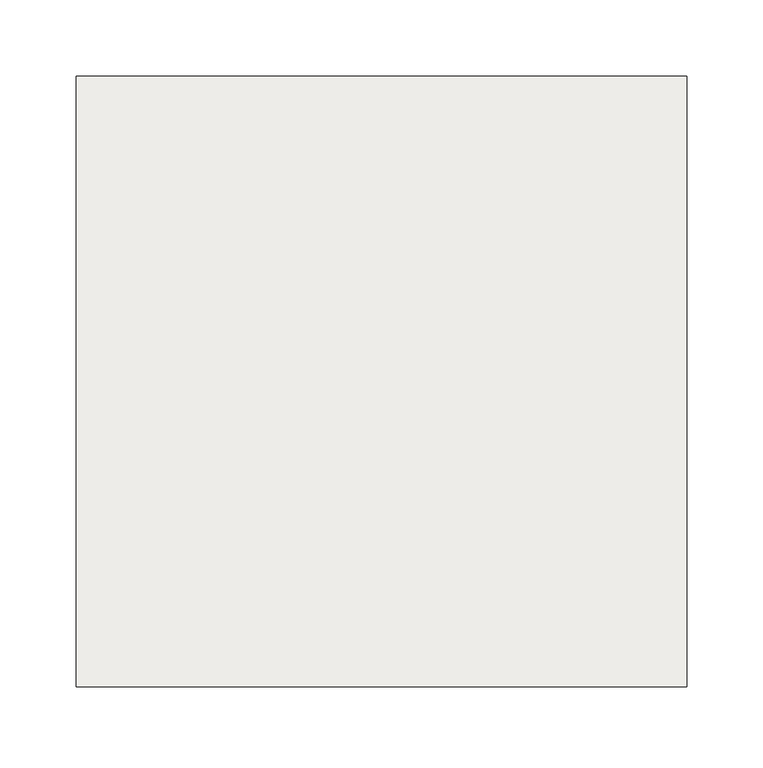
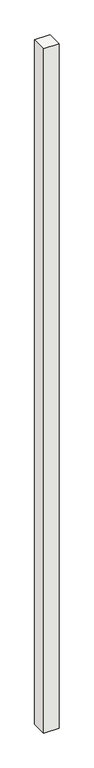
"""IFC4 building model written with IfcOpenShell, lengths in millimetres: footing geometry, NLRS_17_SFO_TLB_funderingspaal geheid beton prefab-AV-MMBPC_gen_rsf : heipaal beton prefab_gen__bxh 400x400."""

from ifc_helpers import new_model, si_unit, frame, origin, place, context, project, spatial, polyline, outline, extrude, source, transform, mapped, element, save


def footing_0d914d5e(model_context):
    return source(origin(), model_context, "Body", "SweptSolid", [
        extrude(outline(polyline([(200.0, -200.0), (-200.0, -200.0), (-200.0, 200.0), (200.0, 200.0), (200.0, -200.0)])), frame((0.0, 0.0, -20000.0), z_axis=(0.0, 0.0, 1.0), x_axis=(1.0, 0.0, 0.0)), (0.0, 0.0, 1.0), 18850.0),
    ])


if __name__ == "__main__":
    model = new_model("IFC4")
    model_context = context("Model", 3, world=origin())
    ifc_project = project(units=[si_unit("LENGTHUNIT", "METRE", prefix="MILLI")], contexts=[model_context])
    site = spatial("IfcSite", under=ifc_project)
    building = spatial("IfcBuilding", under=site)
    placement = place(None, origin())
    footing_shape = footing_0d914d5e(model_context)
    element("IfcFooting", 1, ObjectType="NLRS_17_SFO_TLB_funderingspaal geheid beton prefab-AV-MMBPC_gen_rsf : heipaal beton prefab_gen__bxh 400x400", at=placement, inside=building, context=model_context, shape_type="MappedRepresentation", body=[
        mapped(footing_shape, transform((0.0, 0.0, 0.0), x_axis=(1.0, 0.0, 0.0), y_axis=(0.0, 1.0, 0.0), z_axis=(0.0, 0.0, 1.0))),
    ])
    save(model, "model.ifc")

# Revit data of these elements
# Type "NLRS_17_SFO_TLB_funderingspaal geheid beton prefab-AV-MMBPC_gen_rsf : heipaal beton prefab_gen__bxh 400x400"
#   IfcExportAs = "IfcPile"
#   Type Comments = "prefab heipaal 400x400"
#   Model = " "
#   Manufacturer = " "
#   Description = "prefab heipaal 400x400"
#   Assembly Code = "17.21"
#   Width = 400 mm
#   Slanted Angle [instance default] = 0.00°
#   NLRS_S_draagvermogen_trek [instance default] = 0.00 kN
#   NLRS_S_draagvermogen_druk [instance default] = 0.00 kN
#   NLRS_C_lengte [instance default] = 1660 mm
#   NLRS_C_hoogte = 400 mm
#   NLRS_C_breedte = 400 mm
#   Height [instance default] = 1660 mm
#   Length [instance default] = 1660 mm
#   Angle [instance default] = 0.00°
#   Slanted [instance default] = 0
#   Structural Material = NLRS_f2_beton prefab_gen_rsf
#   Keynote = ""
# Element 1 (IfcFooting, "NLRS_17_SFO_TLB_funderingspaal geheid beton prefab-AV-MMBPC_gen_rsf : heipaal beton prefab_gen__bxh 400x400")
#   NLRS_C_lengte = 18850 mm
#   Height = 18850 mm
#   Length = 18850 mm
#   Materials on its faces: "NLRS_f2_beton prefab_gen_rsf"
# Materials
#   "NLRS_f2_beton prefab_gen_rsf": class "F - Niet gebakken kunststeen", colour RGB 129 133 118, transparency 0, Keynote = "f2", Manufacturer = "Revit Standards Foundation", URL = "www.revitstandards.org", Description = "beton prefab", Cost = 0
